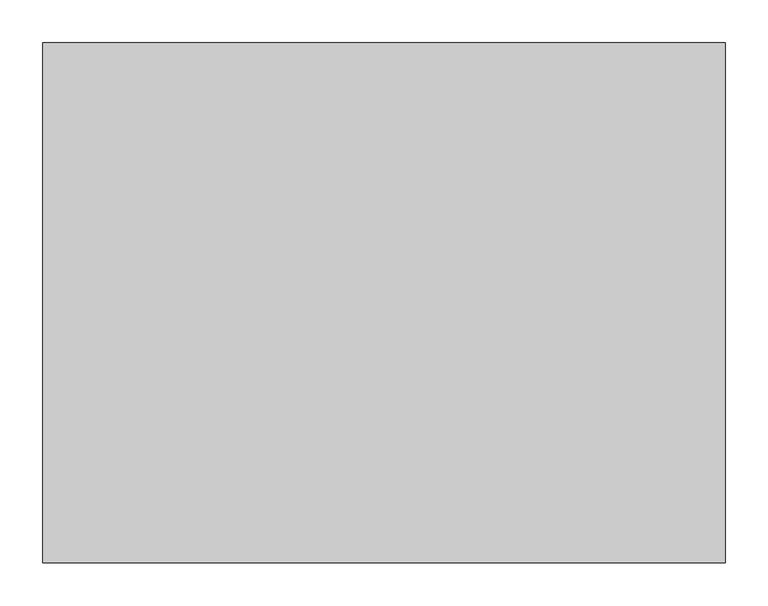
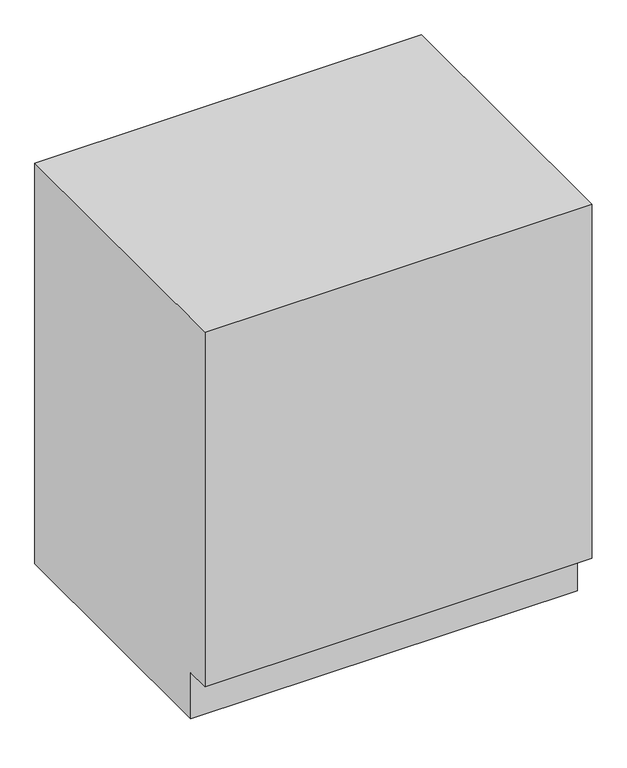
"""IFC4 building model written with IfcOpenShell, lengths in millimetres: furniture geometry, Cabinet, Base Doors and Drawers-NON-COLLECTUS : -."""

from ifc_helpers import new_model, si_unit, frame, origin, place, context, project, spatial, polyline, outline, extrude, source, transform, mapped, element, save


def furniture_d06f3e9b(model_context):
    return source(origin(), model_context, "Body", "SweptSolid", [
        extrude(outline(polyline([(1384.3, 876.2982474), (1993.8987808, 876.2982474), (1993.8987808, 0.0), (1435.1, 0.0), (1435.1, 101.6), (1384.3, 101.6), (1384.3, 876.2982474)])), frame((114.3, 0.0, 0.0), z_axis=(1.0, 0.0, 0.0), x_axis=(0.0, 1.0, 0.0)), (0.0, 0.0, 1.0), 799.9984),
    ])


if __name__ == "__main__":
    model = new_model("IFC4")
    model_context = context("Model", 3, world=origin())
    ifc_project = project(units=[si_unit("LENGTHUNIT", "METRE", prefix="MILLI")], contexts=[model_context])
    site = spatial("IfcSite", under=ifc_project)
    building = spatial("IfcBuilding", under=site)
    placement = place(None, origin())
    furniture_shape = furniture_d06f3e9b(model_context)
    element("IfcFurniture", 1, ObjectType="Cabinet, Base Doors and Drawers-NON-COLLECTUS : -", at=placement, inside=building, context=model_context, shape_type="MappedRepresentation", body=[
        mapped(furniture_shape, transform((0.0, 0.0, 0.0), x_axis=(1.0, 0.0, 0.0), y_axis=(0.0, 1.0, 0.0), z_axis=(0.0, 0.0, 1.0))),
    ])
    save(model, "model.ifc")

# Revit data of these elements
# Type "Cabinet, Base Doors and Drawers-NON-COLLECTUS : -"
#   External ID [instance default] = ""
#   Width Reporting [instance default] = 762 mm
#   Width [instance default] = 762 mm
#   Toe Kick Height = 101.6 mm
#   Toe Kick Depth = 50.8 mm
#   Height of Drawers = 152.4 mm
#   Height Reporting [instance default] = 825.5 mm
#   Height [instance default] = 825.5 mm
#   Depth Reporting [instance default] = 609.6 mm
#   Depth [instance default] = 609.6 mm
#   Material = White
#   Default Elevation = 0
# Element 1 (IfcFurniture, "Cabinet, Base Doors and Drawers-NON-COLLECTUS : -")
#   Width Reporting = 799.998 mm
#   Width = 799.998 mm
#   Height Reporting = 876.298 mm
#   Height = 876.298 mm
#   Depth Reporting = 609.599 mm
#   Depth = 609.599 mm
#   Materials on its faces: "White"
# Materials
#   "White": class "Generic", colour RGB 255 255 255, transparency 0, Cost = 0
